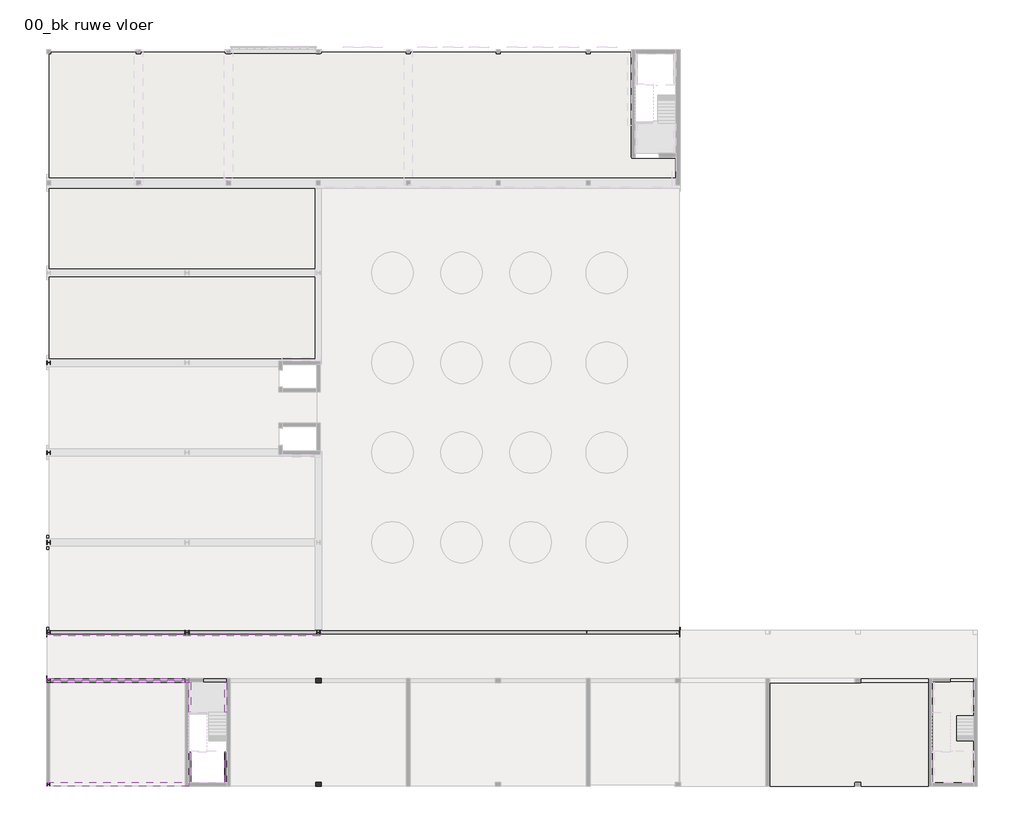
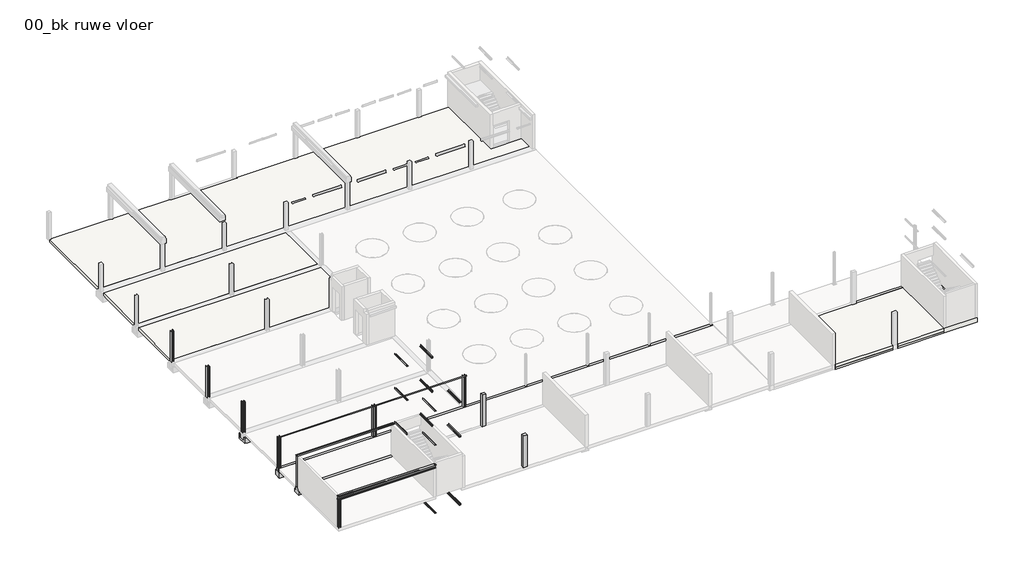
# One storey, part 4 of 6: 24 beams, 10 columns, 8 slabs.
# Revit data of these elements (continued)
# Type "NLRS_28_SF_LIB_stalen ligger stripstaal-AV-MMBS-SRP_gen_rsf : stalen ligger stripstaal RECT_gen__120x15" (continued)
#   vpy = 60 mm
#   NLRS_C_lengte [instance default] = 1500 mm
#   Length [instance default] = 1500 mm
#   bf = 120 mm
#   d = 15 mm
#   Structural Material = NLRS_h2_staal_gen_rsf
#   Keynote = ""
# Type "NLRS_28_SF_LIB_stalen ligger hoekprofiel gelijkzijdig-AV-MMBS-SRP_gen_rsf : stalen ligger gelijkzijdig hoekprofiel LEQU_gen__150x150x15"
#   Export Type to IFC As = "IfcBeamType"
#   Type IfcGUID = "2CEqVLPNH8KRN7ghwV3a1U"
#   Type Comments = "L150x150x15"
#   Model = " "
#   Manufacturer = " "
#   Fire Rating = " "
#   Description = "stalen ligger L150x150x15"
#   Assembly Code = "28.11"
#   vz = 107.5 mm
#   vy = 107.5 mm
#   tw = 15 mm
#   tf = 15 mm
#   ri = 8 mm
#   ra = 16 mm
#   d = 150 mm
#   bf = 150 mm
#   NLRS_C_lengte [instance default] = 1524 mm
#   Length [instance default] = 1524 mm
#   Structural Material = NLRS_h2_staal_gen_rsf
#   Keynote = ""
# Type "NLRS_28_SCO_TLB_stalen kolom HEA-BCPG-MMBS-SRP_gen_rsf : stalen kolom_gen__HEA 260"
#   Type IFC Predefined Type = "COLUMN"
#   Export Type to IFC As = "IfcColumnType"
#   Type IfcGUID = "2$hNzCXOT3YR8V$0CfyzGd"
#   Type Comments = "HEA260"
#   Model = " "
#   Manufacturer = " "
#   Description = "stalen kolom HEA260"
#   Assembly Code = "28.11"
#   vz = 125 mm
#   vy = 130 mm
#   vpz = 125 mm
#   vpy = 130 mm
#   tw = 7.5 mm
#   tf = 12.5 mm
#   ra = 24 mm
#   d = 250 mm
#   bf = 260 mm
#   NLRS_C_lengte [instance default] = 2743.2 mm
#   Structural Material = NLRS_h2_staal_gen_rsf
#   Keynote = ""
# Type "NLRS_28_SCO_TLB_stalen kolom HEB-BCPG-MMBS-SRP_gen_rsf : stalen kolom_gen__HEB 300"
#   Type IFC Predefined Type = "COLUMN"
#   Export Type to IFC As = "IfcColumnType"
#   Type IfcGUID = "3C_b5Xdrv818Ti1jf59K4n"
#   Type Comments = "HEB300"
#   Model = " "
#   Manufacturer = " "
#   Description = "stalen kolom HEB300"
#   Assembly Code = "28.11"
#   vz = 150 mm
#   vy = 150 mm
#   vpz = 150 mm
#   vpy = 150 mm
#   tw = 11 mm
#   tf = 19 mm
#   ra = 27 mm
#   d = 300 mm
#   bf = 300 mm
#   NLRS_C_lengte [instance default] = 2743.2 mm
#   Structural Material = NLRS_h2_staal_gen_rsf
#   Keynote = ""
# Type "NLRS_28_SCO_TLB_vierkante kolom beton ihwg-BCPG-MMBC-SRP_gen_rsf : vierkante kolom beton ihwg_gen__bxh 400x300"
#   Type IFC Predefined Type = "COLUMN"
#   Export Type to IFC As = "IfcColumnType"
#   Type IfcGUID = "2lw04Qbvr9TgC3fLWwYn2N"
#   Type Comments = "400x300"
#   Model = "LOD300"
#   Description = "betonkolom ihwg 400x300"
#   Assembly Code = "28.11"
#   NLRS_C_lengte [instance default] = 2700 mm
#   NLRS_C_hoogte = 300 mm
#   NLRS_C_breedte = 400 mm
#   Structural Material = NLRS_f2_beton ihwg_gen_rsf
# Type "NLRS_28_SCO_TLB_stalen kolom HEA-BCPG-MMBS-SRP_gen_rsf : stalen kolom_gen__HEA 240"
#   Type IFC Predefined Type = "COLUMN"
#   Export Type to IFC As = "IfcColumnType"
#   Type IfcGUID = "2$hNzCXOT3YR8V$0CfyzVH"
#   Type Comments = "HEA240"
#   Model = " "
#   Manufacturer = " "
#   Description = "stalen kolom HEA240"
#   Assembly Code = "28.11"
#   vz = 115 mm
#   vy = 120 mm
#   vpz = 115 mm
#   vpy = 120 mm
#   tw = 7.5 mm
#   tf = 12 mm
#   ra = 21 mm
#   d = 230 mm
#   bf = 240 mm
#   NLRS_C_lengte [instance default] = 2743.2 mm
#   Structural Material = NLRS_h2_staal_gen_rsf
#   Keynote = ""
# Type "NLRS_28_SCO_TLB_stalen kolom HEA-BCPG-MMBS-SRP_gen_rsf : stalen kolom_gen__HEA 200"
#   Type IFC Predefined Type = "COLUMN"
#   Export Type to IFC As = "IfcColumnType"
#   Type IfcGUID = "2$hNzCXOT3YR8V$0CfyzVT"
#   Type Comments = "HEA200"
#   Model = " "
#   Manufacturer = " "
#   Description = "stalen kolom HEA200"
#   Assembly Code = "28.11"
#   vz = 95 mm
#   vy = 100 mm
#   vpz = 95 mm
#   vpy = 100 mm
#   tw = 6.5 mm
#   tf = 10 mm
#   ra = 18 mm
#   d = 190 mm
#   bf = 200 mm
#   NLRS_C_lengte [instance default] = 2743.2 mm
#   Structural Material = NLRS_h2_staal_gen_rsf
#   Keynote = ""
# Type "NLRS_23_FL_isolatieplaatvloer 320_gen_rsf"
#   Keynote = ""
#   Export Type to IFC As = "IfcSlab"
#   Type IfcGUID = "0X0KViByb4JPBOa4XaNeBK"
#   Type Comments = "d=320mm"
#   Description = "prefab isolatieplaatvloer, vrijdragend"
#   Assembly Code = "23.21"
#   Function = 0
#   Layers, outside or top first: 40 mm "NLRS_f2_beton prefab_gen_rsf" (function 1); 235 mm "NLRS_f2_beton prefab_gen_rsf" (function 1); 45 mm "NLRS_f2_beton prefab_gen_rsf" (function 1)
# Type "NLRS_23_FL_beton ihwg vloeraanstort 520_gen_rsf"
#   Keynote = ""
#   Export Type to IFC As = "IfcSlab"
#   Type IfcGUID = "3aMdMHoe12P9KDGPyaIe$w"
#   Type Comments = "vloeraanstort d=520"
#   Description = "in het werk gestorte betonvloer, vrijdragend"
#   Assembly Code = "23.21"
#   Function = 0
#   Layers, outside or top first: 520 mm "NLRS_f2_beton ihwg_gen_rsf" (function 1)
# Type "NLRS_23_FL_isolatie isolatieplaatvloer 200_gen_rsf"
#   Keynote = ""
#   Export Type to IFC As = "IfcSlab"
#   Type IfcGUID = "3aMdMHoe12P9KDGPyaIfI8"
#   Type Comments = "d=200mm"
#   Description = "prefab isolatieplaatvloer, vrijdragend"
#   Assembly Code = "23.21"
#   Function = 0
#   Layers, outside or top first: 200 mm "NLRS_n7_isolatie EPS_gen_rsf" (function 1)
# Element 1 (IfcBeam, "NLRS_28_SF_LIB_balk dubbele sponning beton prefab-CWV-MMBC-SRP_gen_rsf : balk beton prefab_gen__bxh 700x900 met inkassing bxh 200x320")
#   IfcGUID = "0AFZSao6j3uApvehgmz3cS"
#   NLRS_C_lengte = 45800 mm
#   IsExternal = yes
#   LoadBearing = yes
#   Phase Created = NLRS_nieuw
#   Materials on its faces: "NLRS_f2_beton prefab_gen_rsf"
# Element 2 (IfcBeam, "NLRS_28_SF_LIB_balkbodem beton prefab-CWV-MMBC-SRP_gen_rsf : balkbodem beton prefab_gen__bxhxdk 1000x580x200")
#   IfcGUID = "0X0KViByb4JPBOa4XaNgPp"
#   NLRS_C_lengte = 19200 mm
#   IsExternal = yes
#   LoadBearing = yes
#   Phase Created = NLRS_nieuw
#   Materials on its faces: "NLRS_f2_beton prefab_gen_rsf"
# Element 3 (IfcBeam, "NLRS_28_SF_LIB_balk dubbele sponning beton prefab-CWV-MMBC-SRP_gen_rsf : balk beton prefab_gen__bxh 700x700 met inkassing bxh 200x320")
#   IfcGUID = "1pBmRfcsbA7BE9s_rekBS$"
#   NLRS_C_lengte = 10150 mm
#   IsExternal = yes
#   LoadBearing = yes
#   Phase Created = NLRS_nieuw
#   Materials on its faces: "NLRS_f2_beton prefab_gen_rsf", "NLRS_f2_beton ihwg_gen_rsf"
# Element 4 (IfcBeam, "NLRS_28_SF_LIB_balk dubbele sponning beton prefab-CWV-MMBC-SRP_gen_rsf : balk beton prefab_gen__bxh 700x700 met inkassing bxh 200x320")
#   IfcGUID = "1pBmRfcsbA7BE9s_rekB42"
#   NLRS_C_lengte = 2875 mm
#   IsExternal = yes
#   LoadBearing = yes
#   Phase Created = NLRS_nieuw
#   Materials on its faces: "NLRS_f2_beton prefab_gen_rsf"
# Element 5 (IfcBeam, "NLRS_28_SF_LIB_stalen ligger HEB-AV-CWV-MMBS-SRP_gen_rsf : stalen ligger_gen__HEB 360")
#   IfcGUID = "00ECIG4lbEgBwDs3wwpaJg"
#   Comments = ""
#   NLRS_C_lengte = 10275 mm
#   IsExternal = no
#   LoadBearing = yes
#   Phase Created = NLRS_nieuw
#   Materials on its faces: "NLRS_h2_staal_gen_rsf"
# Element 6 (IfcBeam, "NLRS_28_SF_LIB_stalen ligger stripstaal-AV-MMBS-SRP_gen_rsf : stalen ligger stripstaal RECT_gen__140x15")
#   IfcGUID = "00ECIG4lbEgBwDs3wwpaJk"
#   Comments = ""
#   NLRS_C_lengte = 10275 mm
#   IsExternal = no
#   LoadBearing = yes
#   Phase Created = NLRS_nieuw
#   Materials on its faces: "NLRS_h2_staal_gen_rsf"
# Element 7 (IfcBeam, "NLRS_28_SF_LIB_stalen ligger stripstaal-AV-MMBS-SRP_gen_rsf : stalen ligger stripstaal RECT_gen__140x15")
#   IfcGUID = "00ECIG4lbEgBwDs3wwpaJi"
#   Comments = ""
#   NLRS_C_lengte = 10275 mm
#   IsExternal = no
#   LoadBearing = yes
#   Phase Created = NLRS_nieuw
#   Materials on its faces: "NLRS_h2_staal_gen_rsf"
# Element 8 (IfcBeam, "NLRS_28_SF_LIB_stalen ligger stripstaal-AV-MMBS-SRP_gen_rsf : stalen ligger stripstaal RECT_gen__120x15")
#   IfcGUID = "30fJl_yZvFzewSfsmFGxE0"
#   Comments = ""
#   NLRS_C_lengte = 19775 mm
#   IsExternal = no
#   LoadBearing = yes
#   Phase Created = NLRS_nieuw
#   Materials on its faces: "NLRS_h2_staal_gen_rsf"
# Element 9 (IfcBeam, "NLRS_28_SF_LIB_stalen ligger hoekprofiel gelijkzijdig-AV-MMBS-SRP_gen_rsf : stalen ligger gelijkzijdig hoekprofiel LEQU_gen__150x150x15")
#   IfcGUID = "2CEqVLPNH8KRN7ghwV3a5c"
#   NLRS_C_lengte = 2190 mm
#   IsExternal = no
#   LoadBearing = yes
#   Phase Created = NLRS_nieuw
#   Materials on its faces: "NLRS_h2_staal_gen_rsf"
# Element 10 (IfcBeam, "NLRS_28_SF_LIB_stalen ligger hoekprofiel gelijkzijdig-AV-MMBS-SRP_gen_rsf : stalen ligger gelijkzijdig hoekprofiel LEQU_gen__150x150x15")
#   IfcGUID = "2CEqVLPNH8KRN7ghwV3by5"
#   NLRS_C_lengte = 2190 mm
#   IsExternal = no
#   LoadBearing = yes
#   Phase Created = NLRS_nieuw
#   Materials on its faces: "NLRS_h2_staal_gen_rsf"
# Element 11 (IfcBeam, "NLRS_28_SF_LIB_stalen ligger hoekprofiel gelijkzijdig-AV-MMBS-SRP_gen_rsf : stalen ligger gelijkzijdig hoekprofiel LEQU_gen__150x150x15")
#   IfcGUID = "2CEqVLPNH8KRN7ghwV3by_"
#   NLRS_C_lengte = 2190 mm
#   IsExternal = no
#   LoadBearing = yes
#   Phase Created = NLRS_nieuw
#   Materials on its faces: "NLRS_h2_staal_gen_rsf"
# Element 12 (IfcBeam, "NLRS_28_SF_LIB_stalen ligger hoekprofiel gelijkzijdig-AV-MMBS-SRP_gen_rsf : stalen ligger gelijkzijdig hoekprofiel LEQU_gen__150x150x15")
#   IfcGUID = "2CEqVLPNH8KRN7ghwV3bzN"
#   NLRS_C_lengte = 2190 mm
#   IsExternal = no
#   LoadBearing = yes
#   Phase Created = NLRS_nieuw
#   Materials on its faces: "NLRS_h2_staal_gen_rsf"
# Element 13 (IfcBeam, "NLRS_28_SF_LIB_stalen ligger hoekprofiel gelijkzijdig-AV-MMBS-SRP_gen_rsf : stalen ligger gelijkzijdig hoekprofiel LEQU_gen__150x150x15")
#   IfcGUID = "2CEqVLPNH8KRN7ghwV3b_X"
#   NLRS_C_lengte = 2190 mm
#   IsExternal = no
#   LoadBearing = yes
#   Phase Created = NLRS_nieuw
#   Materials on its faces: "NLRS_h2_staal_gen_rsf"
# Element 14 (IfcBeam, "NLRS_28_SF_LIB_stalen ligger hoekprofiel gelijkzijdig-AV-MMBS-SRP_gen_rsf : stalen ligger gelijkzijdig hoekprofiel LEQU_gen__150x150x15")
#   IfcGUID = "2CEqVLPNH8KRN7ghwV3baI"
#   NLRS_C_lengte = 2190 mm
#   IsExternal = no
#   LoadBearing = yes
#   Phase Created = NLRS_nieuw
#   Materials on its faces: "NLRS_h2_staal_gen_rsf"
# Element 15 (IfcBeam, "NLRS_28_SF_LIB_stalen ligger hoekprofiel gelijkzijdig-AV-MMBS-SRP_gen_rsf : stalen ligger gelijkzijdig hoekprofiel LEQU_gen__150x150x15")
#   IfcGUID = "2CEqVLPNH8KRN7ghwV3baB"
#   NLRS_C_lengte = 2190 mm
#   IsExternal = no
#   LoadBearing = yes
#   Phase Created = NLRS_nieuw
#   Materials on its faces: "NLRS_h2_staal_gen_rsf"
# Element 16 (IfcBeam, "NLRS_28_SF_LIB_stalen ligger hoekprofiel gelijkzijdig-AV-MMBS-SRP_gen_rsf : stalen ligger gelijkzijdig hoekprofiel LEQU_gen__150x150x15")
#   IfcGUID = "2CEqVLPNH8KRN7ghwV3bai"
#   NLRS_C_lengte = 2190 mm
#   IsExternal = no
#   LoadBearing = yes
#   Phase Created = NLRS_nieuw
#   Materials on its faces: "NLRS_h2_staal_gen_rsf"
# Element 17 (IfcBeam, "NLRS_28_SF_LIB_stalen ligger hoekprofiel gelijkzijdig-AV-MMBS-SRP_gen_rsf : stalen ligger gelijkzijdig hoekprofiel LEQU_gen__150x150x15")
#   IfcGUID = "2CEqVLPNH8KRN7ghwV3bxp"
#   NLRS_C_lengte = 2190 mm
#   IsExternal = no
#   LoadBearing = yes
#   Phase Created = NLRS_nieuw
#   Materials on its faces: "NLRS_h2_staal_gen_rsf"
# Element 18 (IfcBeam, "NLRS_28_SF_LIB_stalen ligger hoekprofiel gelijkzijdig-AV-MMBS-SRP_gen_rsf : stalen ligger gelijkzijdig hoekprofiel LEQU_gen__150x150x15")
#   IfcGUID = "2CEqVLPNH8KRN7ghwV3by0"
#   NLRS_C_lengte = 2190 mm
#   IsExternal = no
#   LoadBearing = yes
#   Phase Created = NLRS_nieuw
#   Materials on its faces: "NLRS_h2_staal_gen_rsf"
# Element 19 (IfcBeam, "NLRS_28_SF_LIB_stalen ligger hoekprofiel gelijkzijdig-AV-MMBS-SRP_gen_rsf : stalen ligger gelijkzijdig hoekprofiel LEQU_gen__150x150x15")
#   IfcGUID = "2CEqVLPNH8KRN7ghwV3byv"
#   NLRS_C_lengte = 2190 mm
#   IsExternal = no
#   LoadBearing = yes
#   Phase Created = NLRS_nieuw
#   Materials on its faces: "NLRS_h2_staal_gen_rsf"
# Element 20 (IfcBeam, "NLRS_28_SF_LIB_stalen ligger hoekprofiel gelijkzijdig-AV-MMBS-SRP_gen_rsf : stalen ligger gelijkzijdig hoekprofiel LEQU_gen__150x150x15")
#   IfcGUID = "2CEqVLPNH8KRN7ghwV3bzI"
#   NLRS_C_lengte = 2190 mm
#   IsExternal = no
#   LoadBearing = yes
#   Phase Created = NLRS_nieuw
#   Materials on its faces: "NLRS_h2_staal_gen_rsf"
# Element 21 (IfcBeam, "NLRS_28_SF_LIB_stalen ligger hoekprofiel gelijkzijdig-AV-MMBS-SRP_gen_rsf : stalen ligger gelijkzijdig hoekprofiel LEQU_gen__150x150x15")
#   IfcGUID = "2CEqVLPNH8KRN7ghwV3b_i"
#   NLRS_C_lengte = 2190 mm
#   IsExternal = no
#   LoadBearing = yes
#   Phase Created = NLRS_nieuw
#   Materials on its faces: "NLRS_h2_staal_gen_rsf"
# Element 22 (IfcBeam, "NLRS_28_SF_LIB_stalen ligger hoekprofiel gelijkzijdig-AV-MMBS-SRP_gen_rsf : stalen ligger gelijkzijdig hoekprofiel LEQU_gen__150x150x15")
#   IfcGUID = "2CEqVLPNH8KRN7ghwV3baS"
#   NLRS_C_lengte = 2190 mm
#   IsExternal = no
#   LoadBearing = yes
#   Phase Created = NLRS_nieuw
#   Materials on its faces: "NLRS_h2_staal_gen_rsf"
# Element 23 (IfcBeam, "NLRS_28_SF_LIB_stalen ligger hoekprofiel gelijkzijdig-AV-MMBS-SRP_gen_rsf : stalen ligger gelijkzijdig hoekprofiel LEQU_gen__150x150x15")
#   IfcGUID = "2CEqVLPNH8KRN7ghwV3bar"
#   NLRS_C_lengte = 2190 mm
#   IsExternal = no
#   LoadBearing = yes
#   Phase Created = NLRS_nieuw
#   Materials on its faces: "NLRS_h2_staal_gen_rsf"
# Element 24 (IfcBeam, "NLRS_28_SF_LIB_stalen ligger hoekprofiel gelijkzijdig-AV-MMBS-SRP_gen_rsf : stalen ligger gelijkzijdig hoekprofiel LEQU_gen__150x150x15")
#   IfcGUID = "2CEqVLPNH8KRN7ghwV3bak"
#   NLRS_C_lengte = 2190 mm
#   IsExternal = no
#   LoadBearing = yes
#   Phase Created = NLRS_nieuw
#   Materials on its faces: "NLRS_h2_staal_gen_rsf"
# Element 25 (IfcColumn, "NLRS_28_SCO_TLB_stalen kolom HEA-BCPG-MMBS-SRP_gen_rsf : stalen kolom_gen__HEA 260")
#   IfcGUID = "2$hNzCXOT3YR8V$0Cfyz77"
#   Comments = ""
#   IsExternal = no
#   LoadBearing = yes
#   Phase Created = NLRS_nieuw
#   Materials on its faces: "NLRS_h2_staal_gen_rsf"
# Element 26 (IfcColumn, "NLRS_28_SCO_TLB_stalen kolom HEA-BCPG-MMBS-SRP_gen_rsf : stalen kolom_gen__HEA 260")
#   IfcGUID = "2$hNzCXOT3YR8V$0Cfyz53"
#   Comments = ""
#   IsExternal = no
#   LoadBearing = yes
#   Phase Created = NLRS_nieuw
#   Materials on its faces: "NLRS_h2_staal_gen_rsf"
# Element 27 (IfcColumn, "NLRS_28_SCO_TLB_stalen kolom HEA-BCPG-MMBS-SRP_gen_rsf : stalen kolom_gen__HEA 260")
#   IfcGUID = "2$hNzCXOT3YR8V$0Cfyz3A"
#   Comments = ""
#   IsExternal = no
#   LoadBearing = yes
#   Phase Created = NLRS_nieuw
#   Materials on its faces: "NLRS_h2_staal_gen_rsf"
# Element 28 (IfcColumn, "NLRS_28_SCO_TLB_stalen kolom HEA-BCPG-MMBS-SRP_gen_rsf : stalen kolom_gen__HEA 260")
#   IfcGUID = "2$hNzCXOT3YR8V$0Cfyz25"
#   Comments = ""
#   IsExternal = no
#   LoadBearing = yes
#   Phase Created = NLRS_nieuw
#   Materials on its faces: "NLRS_h2_staal_gen_rsf"
# Element 29 (IfcColumn, "NLRS_28_SCO_TLB_stalen kolom HEB-BCPG-MMBS-SRP_gen_rsf : stalen kolom_gen__HEB 300")
#   IfcGUID = "2GRbcre991teoKeCLB8Lxz"
#   Comments = ""
#   IsExternal = no
#   LoadBearing = yes
#   Phase Created = NLRS_nieuw
#   Materials on its faces: "NLRS_h2_staal_gen_rsf"
# Element 30 (IfcColumn, "NLRS_28_SCO_TLB_stalen kolom HEA-BCPG-MMBS-SRP_gen_rsf : stalen kolom_gen__HEA 260")
#   IfcGUID = "2GRbcre991teoKeCLB8Lws"
#   Comments = ""
#   IsExternal = no
#   LoadBearing = yes
#   Phase Created = NLRS_nieuw
#   Materials on its faces: "NLRS_h2_staal_gen_rsf"
# Element 31 (IfcColumn, "NLRS_28_SCO_TLB_vierkante kolom beton ihwg-BCPG-MMBC-SRP_gen_rsf : vierkante kolom beton ihwg_gen__bxh 400x300")
#   IfcGUID = "2lw04Qbvr9TgC3fLWwYnCj"
#   IsExternal = no
#   LoadBearing = yes
#   Phase Created = NLRS_nieuw
#   Materials on its faces: "NLRS_f2_beton ihwg_gen_rsf"
# Element 32 (IfcColumn, "NLRS_28_SCO_TLB_vierkante kolom beton ihwg-BCPG-MMBC-SRP_gen_rsf : vierkante kolom beton ihwg_gen__bxh 400x300")
#   IfcGUID = "2lw04Qbvr9TgC3fLWwYn7v"
#   IsExternal = no
#   LoadBearing = yes
#   Phase Created = NLRS_nieuw
#   Materials on its faces: "NLRS_f2_beton ihwg_gen_rsf"
# Element 33 (IfcColumn, "NLRS_28_SCO_TLB_stalen kolom HEA-BCPG-MMBS-SRP_gen_rsf : stalen kolom_gen__HEA 240")
#   IfcGUID = "00ECIG4lbEgBwDs3wwpb$e"
#   Comments = ""
#   IsExternal = no
#   LoadBearing = yes
#   Phase Created = NLRS_nieuw
#   Materials on its faces: "NLRS_h2_staal_gen_rsf"
# Element 34 (IfcColumn, "NLRS_28_SCO_TLB_stalen kolom HEA-BCPG-MMBS-SRP_gen_rsf : stalen kolom_gen__HEA 200")
#   IfcGUID = "00ECIG4lbEgBwDs3wwpbsp"
#   Comments = ""
#   IsExternal = no
#   LoadBearing = yes
#   Phase Created = NLRS_nieuw
#   Materials on its faces: "NLRS_h2_staal_gen_rsf"
# Element 35 (IfcSlab, "NLRS_23_FL_isolatieplaatvloer 320_gen_rsf")
#   IfcGUID = "2bNskL0kfByRmbY5G6IfIf"
#   built-in parameter 1001955 = 1.5708 (stored number, unit not read)
#   Height Offset From Level = 0 mm
#   built-in parameter 1001954 = 1
#   IsExternal = yes
#   LoadBearing = yes
#   Phase Created = NLRS_nieuw
#   Materials on its faces: "NLRS_f2_beton prefab_gen_rsf"
# Element 36 (IfcSlab, "NLRS_23_FL_isolatieplaatvloer 320_gen_rsf")
#   IfcGUID = "2bNskL0kfByRmbY5G6IfNQ"
#   built-in parameter 1001955 = 1.5708 (stored number, unit not read)
#   Height Offset From Level = 0 mm
#   built-in parameter 1001954 = 1
#   IsExternal = yes
#   LoadBearing = yes
#   Phase Created = NLRS_nieuw
#   Materials on its faces: "NLRS_f2_beton prefab_gen_rsf"
# Element 37 (IfcSlab, "NLRS_23_FL_isolatieplaatvloer 320_gen_rsf")
#   IfcGUID = "1E6t7WhRf97hJGfj3Bm3pQ"
#   Comments = ""
#   built-in parameter 1001955 = -1.5708 (stored number, unit not read)
#   Height Offset From Level = 0 mm
#   built-in parameter 1001954 = 1
#   IsExternal = yes
#   LoadBearing = yes
#   Phase Created = NLRS_nieuw
#   Materials on its faces: "NLRS_f2_beton prefab_gen_rsf"
# Element 38 (IfcSlab, "NLRS_23_FL_isolatieplaatvloer 320_gen_rsf")
#   IfcGUID = "2gNlyDOFb5qwP_T4qK0dKx"
#   Comments = ""
#   built-in parameter 1001955 = -1.5708 (stored number, unit not read)
#   Height Offset From Level = 0 mm
#   built-in parameter 1001954 = 1
#   IsExternal = yes
#   LoadBearing = yes
#   Phase Created = NLRS_nieuw
#   Materials on its faces: "NLRS_f2_beton prefab_gen_rsf"
# Element 39 (IfcSlab, "NLRS_23_FL_isolatieplaatvloer 320_gen_rsf")
#   IfcGUID = "0H0z87ABnEyOuaeN1efimG"
#   Comments = ""
#   built-in parameter 1001955 = 1.5708 (stored number, unit not read)
#   Height Offset From Level = 0 mm
#   built-in parameter 1001954 = 1
#   IsExternal = yes
#   LoadBearing = yes
#   Phase Created = NLRS_nieuw
#   Materials on its faces: "NLRS_f2_beton prefab_gen_rsf"
# Element 40 (IfcSlab, "NLRS_23_FL_beton ihwg vloeraanstort 520_gen_rsf")
#   IfcGUID = "3aMdMHoe12P9KDGPyaIeY6"
#   Height Offset From Level = 0 mm
#   built-in parameter 1001954 = 1
#   IsExternal = yes
#   LoadBearing = yes
#   Phase Created = NLRS_nieuw
#   Materials on its faces: "NLRS_f2_beton ihwg_gen_rsf"
# Element 41 (IfcSlab, "NLRS_23_FL_isolatie isolatieplaatvloer 200_gen_rsf")
#   IfcGUID = "3aMdMHoe12P9KDGPyaIfHv"
#   built-in parameter 1001955 = 1.5708 (stored number, unit not read)
#   Height Offset From Level = -320 mm
#   built-in parameter 1001954 = 1
#   IsExternal = yes
#   LoadBearing = yes
#   Phase Created = NLRS_nieuw
#   Materials on its faces: "NLRS_n7_isolatie EPS_gen_rsf"
# Element 42 (IfcSlab, "NLRS_23_FL_isolatie isolatieplaatvloer 200_gen_rsf")
#   IfcGUID = "3aMdMHoe12P9KDGPyaIfLI"
#   built-in parameter 1001955 = 1.5708 (stored number, unit not read)
#   Height Offset From Level = -320 mm
#   built-in parameter 1001954 = 1
#   IsExternal = yes
#   LoadBearing = yes
#   Phase Created = NLRS_nieuw
#   Materials on its faces: "NLRS_n7_isolatie EPS_gen_rsf"
# Materials
#   "NLRS_f2_beton prefab_gen_rsf": class "F - Niet gebakken kunststeen", colour RGB 129 133 118, transparency 0, Keynote = "f2", Manufacturer = "Revit Standards Foundation", URL = "www.revitstandards.org", Description = "beton prefab", Cost = 0
#   "NLRS_h2_staal_gen_rsf": class "H - Metaal", colour RGB 189 187 185, transparency 0, Keynote = "h2", Manufacturer = "Revit Standards Foundation", URL = "www.revitstandards.org", Description = "staal", Cost = 0
#   "NLRS_f2_beton ihwg_gen_rsf": class "F - Niet gebakken kunststeen", colour RGB 129 133 118, transparency 0, Keynote = "f2", Manufacturer = "Revit Standards Foundation", URL = "www.revitstandards.org", Description = "beton ihwg", Cost = 0
#   "NLRS_n7_isolatie EPS_gen_rsf": class "N - Kunststoffen, rubbers", colour RGB 200 200 140, transparency 0, Keynote = "n7", Manufacturer = "Revit Standards Foundation", URL = "www.revitstandards.org", Description = "isolatie EPS", Cost = 0
